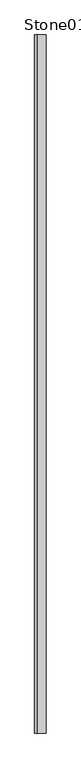
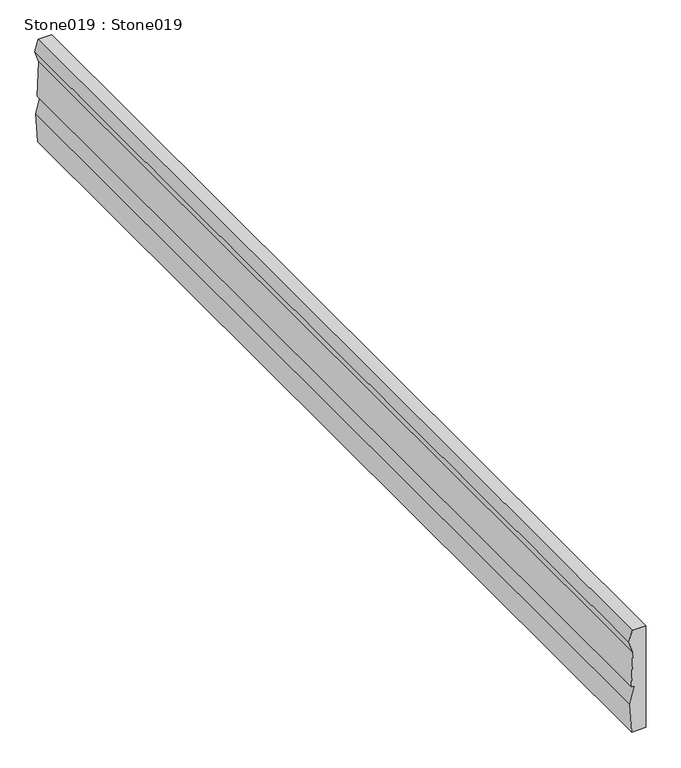
"""IFC4 building model written with IfcOpenShell, lengths in millimetres: proxy geometry, Stone019 : Stone019."""

from ifc_helpers import new_model, si_unit, frame, origin, place, context, project, spatial, polyline, outline, extrude, source, transform, mapped, element, save


def stone019_stone019_5f771642(model_context):
    return source(origin(), model_context, "Body", "SweptSolid", [
        extrude(outline(polyline([(33176.3632813, -10292.7626953), (33153.1347246, -10298.9867683), (33130.484375, -10291.4746094), (33060.5703125, -10294.4003906), (33059.2695313, -10288.8720703), (33025.4492188, -10297.0029297), (32966.9257813, -10293.4648437), (32966.9257813, -10266.1494141), (33176.3632813, -10266.1494141), (33176.3632813, -10292.7626953)])), frame((0.0, 7982.1531721, 0.0), z_axis=(0.0, 1.0, 0.0), x_axis=(0.0, 0.0, 1.0)), (0.0, 0.0, 1.0), 2000.0),
    ])


if __name__ == "__main__":
    model = new_model("IFC4")
    model_context = context("Model", 3, world=origin())
    ifc_project = project(units=[si_unit("LENGTHUNIT", "METRE", prefix="MILLI")], contexts=[model_context])
    site = spatial("IfcSite", under=ifc_project)
    building = spatial("IfcBuilding", under=site)
    placement = place(None, origin())
    stone019_stone019_shape = stone019_stone019_5f771642(model_context)
    element("IfcBuildingElementProxy", 1, Name="Stone019 : Stone019", ObjectType="Stone019 : Stone019", at=placement, inside=building, context=model_context, shape_type="MappedRepresentation", body=[
        mapped(stone019_stone019_shape, transform((0.0, 0.0, 0.0), x_axis=(1.0, 0.0, 0.0), y_axis=(0.0, 1.0, 0.0), z_axis=(0.0, 0.0, 1.0))),
    ])
    save(model, "model.ifc")

# Revit data of these elements
# Type "Stone019 : Stone019"
#   NameOverride = "Stone019"
# Element 1 (IfcBuildingElementProxy, "Stone019 : Stone019")
#   Materials on its faces: "SPLIT FACE STONE 1032"
# Materials
#   "SPLIT FACE STONE 1032": class "Unassigned", colour RGB 205 195 181, transparency 0
